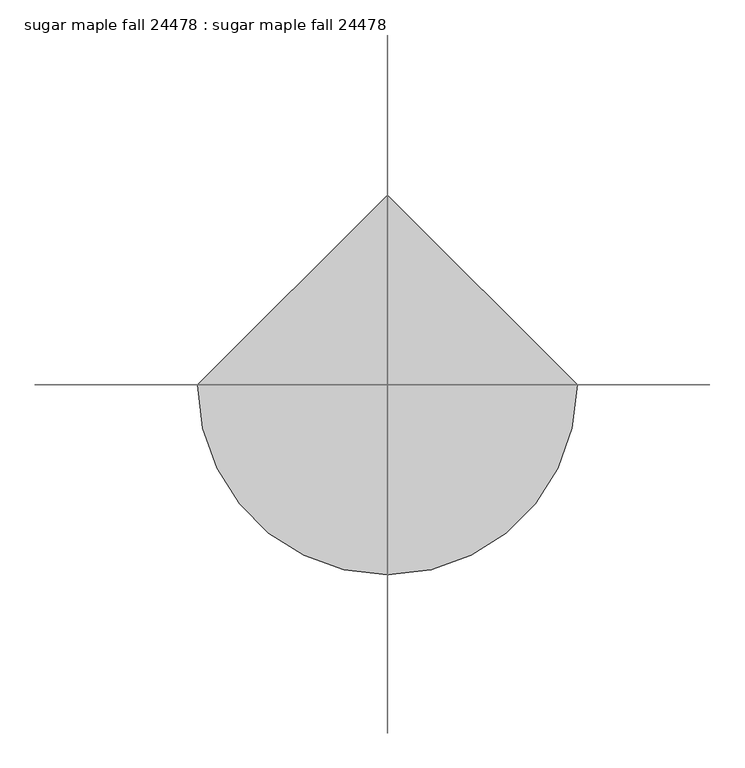
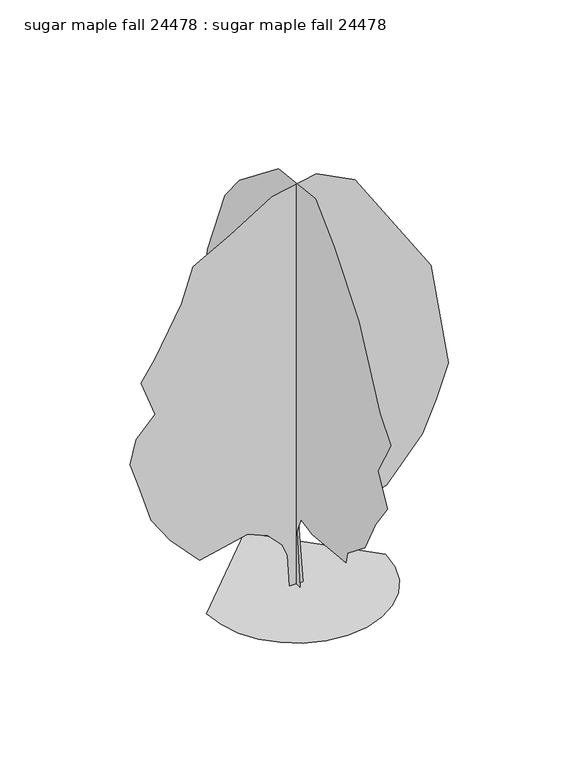
"""IFC4 building model written with IfcOpenShell, lengths in millimetres: proxy geometry, sugar maple fall 24478 : sugar maple fall 24478."""

import ifcopenshell
import ifcopenshell.guid

model = None  # the IFC model being written
_history = None  # IfcOwnerHistory: only IFC2X3 demands one
_inside = {}  # id of a spatial element -> (the spatial element, [elements in it])
_under = {}  # id of a project, library or spatial element -> (it, [spatial elements below it])
_declared = {}  # id of a project -> (the project, [libraries it declares])
_typed = {}  # id of a type object -> (the type object, [elements of that type])
_made_of = {}  # id of a material, layer set ... -> (it, [elements and type objects made of it])


def new_model(schema):
    """Start an empty IFC model of exactly this schema.

    Asked for "IFC4X3", IfcOpenShell would pick the latest addendum, in which some entities
    have other attributes; the version numbers below select the first issue.
    IFC2X3 requires an IfcOwnerHistory on every rooted entity: one is made here for all.
    """
    global model, _history
    if schema == "IFC4X3":
        model = ifcopenshell.file(schema_version=(4, 3, 0, 0))
    else:
        model = ifcopenshell.file(schema=schema)
    _inside.clear()
    _under.clear()
    _declared.clear()
    _typed.clear()
    _made_of.clear()
    _history = None
    if model.schema == "IFC2X3":
        org = make("IfcOrganization", Name="unknown")
        user = make(
            "IfcPersonAndOrganization",
            ThePerson=make("IfcPerson", FamilyName="unknown"),
            TheOrganization=org,
        )
        app = make(
            "IfcApplication",
            ApplicationDeveloper=org,
            Version="unknown",
            ApplicationFullName="unknown",
            ApplicationIdentifier="unknown",
        )
        _history = make(
            "IfcOwnerHistory",
            OwningUser=user,
            OwningApplication=app,
            ChangeAction="ADDED",
            CreationDate=0,
        )
    return model


def make(cls, **values):
    """One entity of the class cls with the attributes given. An attribute that is None is left unset."""
    return model.create_entity(
        cls, **{name: value for name, value in values.items() if value is not None}
    )


def rooted(cls, **values):
    """An entity with a GlobalId (a new one), such as an element, a storey or a relation."""
    return make(cls, GlobalId=ifcopenshell.guid.new(), OwnerHistory=_history, **values)


def si_unit(unit_type, name, prefix=None):
    """IfcSIUnit, for example si_unit("LENGTHUNIT", "METRE", prefix="MILLI")."""
    return make("IfcSIUnit", UnitType=unit_type, Prefix=prefix, Name=name)


def assignment(units):
    """IfcUnitAssignment: the units of a project."""
    return None if units is None else make("IfcUnitAssignment", Units=units)


def point(xyz):
    """IfcCartesianPoint."""
    return None if xyz is None else make("IfcCartesianPoint", Coordinates=xyz)


def direction(xyz):
    """IfcDirection."""
    return None if xyz is None else make("IfcDirection", DirectionRatios=xyz)


def frame(location, z_axis=None, x_axis=None):
    """IfcAxis2Placement3D, a coordinate frame: its origin and axes. An axis left out is left unset."""
    return make(
        "IfcAxis2Placement3D",
        Location=point(location),
        Axis=direction(z_axis),
        RefDirection=direction(x_axis),
    )


def origin():
    """The frame at (0, 0, 0) with its axes left unset."""
    return frame((0.0, 0.0, 0.0))


def place(relative_to, where):
    """IfcLocalPlacement: puts the frame where relative to a parent placement (None: the world)."""
    return make(
        "IfcLocalPlacement", PlacementRelTo=relative_to, RelativePlacement=where
    )


def context(
    kind, dimensions, precision=None, world=None, true_north=None, identifier=None
):
    """IfcGeometricRepresentationContext, for example the 3D "Model" context."""
    return make(
        "IfcGeometricRepresentationContext",
        ContextIdentifier=identifier,
        ContextType=kind,
        CoordinateSpaceDimension=dimensions,
        Precision=precision,
        WorldCoordinateSystem=world,
        TrueNorth=true_north,
    )


def project(units=None, contexts=None):
    """IfcProject with its units and contexts."""
    return rooted(
        "IfcProject",
        Name="project",
        RepresentationContexts=contexts,
        UnitsInContext=assignment(units),
    )


def spatial(cls, under=None, at=None, **own):
    """A site, building, storey or space (cls), placed at a placement, below another one or the project."""
    s = rooted(cls, ObjectPlacement=at, **own)
    if under is not None:
        _under.setdefault(under.id(), (under, []))[1].append(s)
    return s


def point_list(points):
    """IfcCartesianPointList2D or 3D."""
    cls = (
        "IfcCartesianPointList2D" if len(points[0]) == 2 else "IfcCartesianPointList3D"
    )
    return make(cls, CoordList=points)


def triangles(points, corners, closed=None, point_numbers=None):
    """IfcTriangulatedFaceSet: each triangle names its three corners, points numbered from 1."""
    return make(
        "IfcTriangulatedFaceSet",
        Coordinates=point_list(points),
        Closed=closed,
        CoordIndex=corners,
        PnIndex=point_numbers,
    )


def shape(context_of_items, identifier, shape_type, items):
    """IfcShapeRepresentation: the items that make up one representation, for example the "Body"."""
    return make(
        "IfcShapeRepresentation",
        ContextOfItems=context_of_items,
        RepresentationIdentifier=identifier,
        RepresentationType=shape_type,
        Items=items,
    )


def source(mapping_origin, context_of_items, identifier, shape_type, items):
    """IfcRepresentationMap: a shape defined once, which mapped items show again and again."""
    return make(
        "IfcRepresentationMap",
        MappingOrigin=mapping_origin,
        MappedRepresentation=shape(context_of_items, identifier, shape_type, items),
    )


def transform(
    local_origin,
    x_axis=None,
    y_axis=None,
    z_axis=None,
    scale=None,
    scale2=None,
    scale3=None,
    uniform=True,
):
    """IfcCartesianTransformationOperator3D, or its non-uniform kind. x_axis, y_axis, z_axis: its Axis1, 2, 3."""
    if uniform:
        return make(
            "IfcCartesianTransformationOperator3D",
            Axis1=direction(x_axis),
            Axis2=direction(y_axis),
            LocalOrigin=point(local_origin),
            Scale=scale,
            Axis3=direction(z_axis),
        )
    return make(
        "IfcCartesianTransformationOperator3DnonUniform",
        Axis1=direction(x_axis),
        Axis2=direction(y_axis),
        LocalOrigin=point(local_origin),
        Scale=scale,
        Axis3=direction(z_axis),
        Scale2=scale2,
        Scale3=scale3,
    )


def mapped(mapping_source, mapping_target):
    """IfcMappedItem: shows the shape of a source again, moved by a transform."""
    return make(
        "IfcMappedItem", MappingSource=mapping_source, MappingTarget=mapping_target
    )


def made_of(thing, what):
    """Note that an element or type object is made of a material, layer set ...; save() writes the relation."""
    if what is not None:
        _made_of.setdefault(what.id(), (what, []))[1].append(thing)
    return thing


def element(
    cls,
    number,
    at=None,
    inside=None,
    cuts=None,
    type_object=None,
    material=None,
    context=None,
    identifier="Body",
    shape_type=None,
    held_by="IfcProductDefinitionShape",
    body=None,
    shapes=None,
    **own,
):
    """One element of the class cls, such as IfcWall. Its Tag is "e" and its number.

    at: its placement. inside: the storey or other place that contains it. cuts: it is an
    opening in that element (IfcRelVoidsElement). A single representation is given by context,
    identifier, shape_type and body (its items); several are given by shapes. held_by: the class
    of the entity that holds the representations. save() writes the other relations.
    """
    e = rooted(cls, Tag="e%d" % number, ObjectPlacement=at, **own)
    if body is not None:
        shapes = [shape(context, identifier, shape_type, body)]
    if shapes is not None:
        e.Representation = make(held_by, Representations=shapes)
    if inside is not None:
        _inside.setdefault(inside.id(), (inside, []))[1].append(e)
    if cuts is not None:
        rooted(
            "IfcRelVoidsElement", RelatingBuildingElement=cuts, RelatedOpeningElement=e
        )
    if type_object is not None:
        _typed.setdefault(type_object.id(), (type_object, []))[1].append(e)
    return made_of(e, material)


def aggregate(whole, parts):
    """IfcRelAggregates: a whole, such as a stair, and the parts it consists of."""
    return rooted("IfcRelAggregates", RelatingObject=whole, RelatedObjects=parts)


def save(model, path):
    """Write the relations noted so far, then the file.

    IfcRelAggregates (storeys below a building ...), IfcRelContainedInSpatialStructure (elements
    in a storey), IfcRelDefinesByType, IfcRelAssociatesMaterial and IfcRelDeclares: one each for
    every whole, place, type object, material and project.
    """
    for whole, parts in _under.values():
        aggregate(whole, parts)
    for where, things in _inside.values():
        rooted(
            "IfcRelContainedInSpatialStructure",
            RelatedElements=things,
            RelatingStructure=where,
        )
    for kind, things in _typed.values():
        rooted("IfcRelDefinesByType", RelatedObjects=things, RelatingType=kind)
    for what, things in _made_of.values():
        rooted("IfcRelAssociatesMaterial", RelatedObjects=things, RelatingMaterial=what)
    for by, libraries in _declared.values():
        rooted("IfcRelDeclares", RelatingContext=by, RelatedDefinitions=libraries)
    model.write(path)


def sugar_maple_fall_24478_sugar_maple_fall_24478_f594c2a4(model_context):
    return source(origin(), model_context, "Body", "Tessellation", [
        triangles([(-2874.6675568, 0.0, 9.75e-05), (-2798.670742, -658.6848673, 9.75e-05), (-2582.2377319, -1263.582756, 9.75e-05), (-2242.6907249, -1797.3631107, 9.75e-05), (-1797.3631107, -2242.6907249, 9.75e-05), (-1263.582756, -2582.2377319, 9.75e-05), (-658.6848673, -2798.670742, 9.75e-05), (0.0001257, -2874.6675568, 9.75e-05), (658.6848673, -2798.670742, 9.75e-05), (1263.582756, -2582.2377319, 9.75e-05), (1797.3631107, -2242.6907249, 9.75e-05), (2242.6907249, -1797.3631107, 9.75e-05), (2582.2377319, -1263.582756, 9.75e-05), (2798.670742, -658.6848673, 9.75e-05), (2874.6675568, 0.0002513, 9.75e-05), (-0.000377, 2874.6675568, 9.75e-05), (-2.08e-05, -199.1749247, 0.0346819), (4.82e-05, -56.8278721, 1817.6527153), (4.28e-05, -258.825735, 2341.1232342), (-2.85e-05, -903.7539202, 2207.885146), (-0.0001313, -1923.2734486, 2325.3143154), (-0.0002189, -2782.6179428, 2395.771352), (-0.0002163, -2865.4727692, 2771.5436188), (-0.0002948, -3839.4857002, 3546.573056), (-0.0003217, -4426.6312569, 4697.3949623), (-0.000363, -5084.2367569, 5613.3434143), (-0.0002773, -4544.0807739, 6599.7518097), (-0.0003147, -5272.145636, 7891.4671509), (-0.0002294, -4661.5050018, 8619.5320129), (-3.55e-05, -3487.2133072, 11015.1055573), (0.0001602, -2101.5355328, 12729.5788147), (0.0002973, -1068.1552952, 13715.9860474), (0.0005042, 975.1202763, 13504.608252), (0.0006798, 3149.1141769, 11787.0619263), (0.0007341, 3951.829715, 10801.5674286), (0.0007632, 4920.7624329, 8384.6841385), (0.0007481, 5085.151236, 7304.3215942), (0.0007261, 5296.5296127, 5824.7223724), (0.0005924, 4591.9598282, 3804.9162987), (0.0004639, 3629.0215118, 2865.4980583), (0.0004296, 3394.1733467, 2536.687896), (0.000374, 3092.6501816, 1726.1010361), (0.0002152, 1413.0031414, 2273.7472595), (0.0001457, 838.2271059, 1956.0621449), (7.66e-05, 382.876666, 1230.9488468), (2.05e-05, 196.9107642, 0.0347055), (-208.8982774, 9.1e-06, 0.0), (-283.5907205, -0.0001144, 1063.8550489), (-449.8182921, -0.0001567, 1479.347929), (-896.9010681, -0.0001936, 1952.9405331), (-1571.0977066, -0.0001973, 2231.3700497), (-3097.6792351, -8.98e-05, 1888.9910934), (-4045.0475716, -0.0001676, 2888.9678467), (-4666.6866623, -0.0002479, 3790.7939049), (-5023.5305786, -0.0003684, 4932.2431274), (-5340.7001724, -0.0004707, 5906.815036), (-5145.0190933, -0.0005731, 6693.7059586), (-4530.3141724, -0.0006783, 7351.3111679), (-4976.5660034, -0.0008016, 8549.0729416), (-4535.8766235, -0.0009022, 9231.2400238), (-3684.8250824, -0.0011268, 10803.7265991), (-3309.0579025, -0.0012773, 11928.3870209), (-2120.356913, -0.0014059, 12571.4384674), (-772.575808, -0.0015649, 13410.6791016), (660.0640709, -0.0016611, 13692.4909698), (1888.2468075, -0.0016387, 13054.2148132), (4323.8631111, -0.0012977, 9300.6322998), (4887.5394608, -0.0009052, 5801.2272949), (4511.746701, -0.0007572, 4697.3949623), (4053.9121468, -0.0006156, 3677.2051987), (2902.7853172, -0.0004043, 2327.2396339), (1552.5302353, -0.0003087, 2019.9964691), (433.9357224, -0.0003079, 2424.0719501), (75.5588282, -0.0002467, 2041.512743), (218.1486939, -9.5e-06, 0.0310248)], [[15, 16, 1], [14, 15, 1], [14, 1, 2], [13, 14, 2], [13, 2, 3], [13, 3, 4], [12, 13, 4], [11, 12, 4], [11, 4, 5], [11, 5, 6], [11, 6, 7], [11, 7, 8], [11, 8, 9], [11, 9, 10], [46, 17, 18], [45, 46, 18], [44, 45, 18], [41, 42, 43], [44, 18, 19], [21, 22, 23], [27, 28, 29], [25, 26, 27], [31, 32, 33], [31, 33, 34], [30, 31, 34], [30, 34, 35], [30, 35, 36], [29, 30, 36], [27, 29, 36], [27, 36, 37], [25, 27, 37], [24, 25, 37], [23, 24, 37], [21, 23, 37], [20, 21, 37], [19, 20, 37], [19, 37, 38], [19, 38, 39], [19, 39, 40], [19, 40, 41], [19, 41, 43], [44, 19, 43], [74, 75, 47], [74, 47, 48], [74, 48, 49], [74, 49, 50], [51, 52, 53], [58, 59, 60], [61, 62, 63], [73, 74, 50], [73, 50, 51], [51, 53, 54], [51, 54, 55], [73, 51, 55], [73, 55, 56], [73, 56, 57], [73, 57, 58], [73, 58, 60], [73, 60, 61], [73, 61, 63], [73, 63, 64], [73, 64, 65], [73, 65, 66], [73, 66, 67], [73, 67, 68], [73, 68, 69], [73, 69, 70], [73, 70, 71], [73, 71, 72]], closed=False),
    ])


if __name__ == "__main__":
    model = new_model("IFC4")
    model_context = context("Model", 3, world=origin())
    ifc_project = project(units=[si_unit("LENGTHUNIT", "METRE", prefix="MILLI")], contexts=[model_context])
    site = spatial("IfcSite", under=ifc_project)
    building = spatial("IfcBuilding", under=site)
    placement = place(None, origin())
    sugar_maple_fall_24478_sugar_maple_fall_24478_shape = sugar_maple_fall_24478_sugar_maple_fall_24478_f594c2a4(model_context)
    element("IfcBuildingElementProxy", 1, Name="sugar maple fall 24478 : sugar maple fall 24478", ObjectType="sugar maple fall 24478 : sugar maple fall 24478", at=placement, inside=building, context=model_context, shape_type="MappedRepresentation", body=[
        mapped(sugar_maple_fall_24478_sugar_maple_fall_24478_shape, transform((0.0, 0.0, 0.0), x_axis=(1.0, 0.0, 0.0), y_axis=(0.0, 1.0, 0.0), z_axis=(0.0, 0.0, 1.0))),
    ])
    save(model, "model.ifc")

# Revit data of these elements
# Type "sugar maple fall 24478 : sugar maple fall 24478"
#   built-in parameter 1005195 = "RPC-16-FWM4-JJQ0-CAW1-2000-ST1L-LVER-AU"
#   Height = 0
